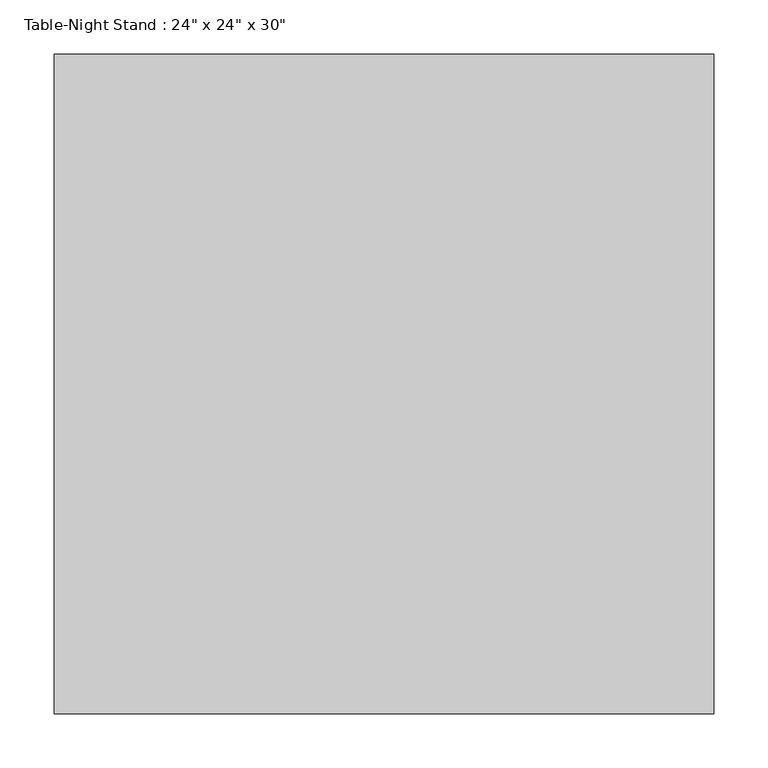
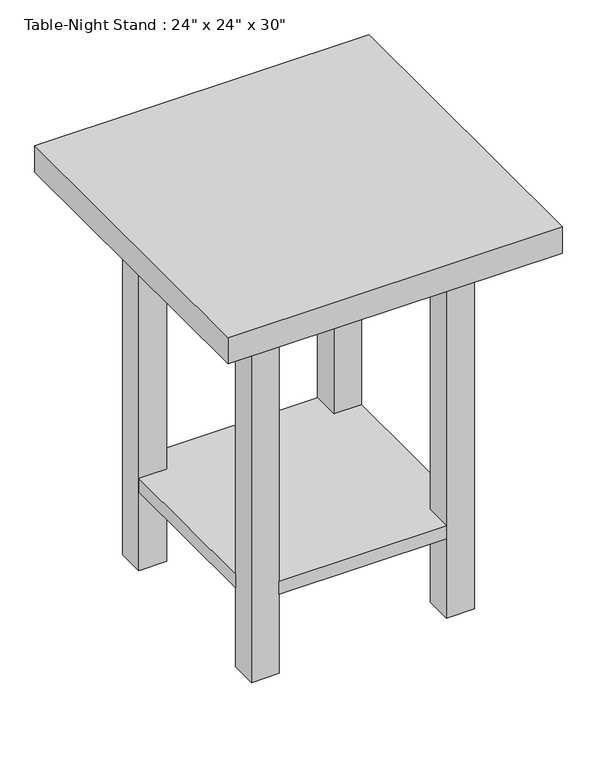
"""IFC4 building model written with IfcOpenShell, lengths in millimetres: furniture geometry."""

from ifc_helpers import new_model, si_unit, frame, origin, origin_with_axes, place, context, project, spatial, polyline, outline, extrude, source, transform, mapped, element, save


def furniture_5bc9ed15(model_context):
    return source(origin(), model_context, "Body", "SweptSolid", [
        extrude(outline(polyline([(156.1336303, 508.0), (460.9336303, 508.0), (460.9336303, 457.2), (511.7336303, 457.2), (511.7336303, 152.4), (460.9336303, 152.4), (460.9336303, 101.6), (156.1336303, 101.6), (156.1336303, 152.4), (105.3336303, 152.4), (105.3336303, 457.2), (156.1336303, 457.2), (156.1336303, 508.0)])), frame((0.0, 0.0, 152.4), z_axis=(0.0, 0.0, 1.0), x_axis=(1.0, 0.0, 0.0)), (0.0, 0.0, 1.0), 25.4),
        extrude(outline(polyline([(156.1336303, 508.0), (156.1336303, 457.2), (105.3336303, 457.2), (105.3336303, 508.0), (156.1336303, 508.0)])), origin_with_axes(), (0.0, 0.0, 1.0), 711.2),
        extrude(outline(polyline([(156.1336303, 152.4), (156.1336303, 101.6), (105.3336303, 101.6), (105.3336303, 152.4), (156.1336303, 152.4)])), origin_with_axes(), (0.0, 0.0, 1.0), 711.2),
        extrude(outline(polyline([(511.7336303, 508.0), (511.7336303, 457.2), (460.9336303, 457.2), (460.9336303, 508.0), (511.7336303, 508.0)])), origin_with_axes(), (0.0, 0.0, 1.0), 711.2),
        extrude(outline(polyline([(511.7336303, 152.4), (511.7336303, 101.6), (460.9336303, 101.6), (460.9336303, 152.4), (511.7336303, 152.4)])), origin_with_axes(), (0.0, 0.0, 1.0), 711.2),
        extrude(outline(polyline([(613.3336303, 0.0), (3.7336303, 0.0), (3.7336303, 609.6), (613.3336303, 609.6), (613.3336303, 0.0)])), frame((0.0, 0.0, 711.2), z_axis=(0.0, 0.0, 1.0), x_axis=(1.0, 0.0, 0.0)), (0.0, 0.0, 1.0), 50.8),
    ])


if __name__ == "__main__":
    model = new_model("IFC4")
    model_context = context("Model", 3, world=origin())
    ifc_project = project(units=[si_unit("LENGTHUNIT", "METRE", prefix="MILLI")], contexts=[model_context])
    site = spatial("IfcSite", under=ifc_project)
    building = spatial("IfcBuilding", under=site)
    placement = place(None, origin())
    furniture_shape = furniture_5bc9ed15(model_context)
    element("IfcFurniture", 1, ObjectType="Table-Night Stand : 24\" x 24\" x 30\"", at=placement, inside=building, context=model_context, shape_type="MappedRepresentation", body=[
        mapped(furniture_shape, transform((0.0, 0.0, 0.0), x_axis=(1.0, 0.0, 0.0), y_axis=(0.0, 1.0, 0.0), z_axis=(0.0, 0.0, 1.0))),
    ])
    save(model, "model.ifc")

# Revit data of these elements
# Type "Table-Night Stand : 24\" x 24\" x 30\""
#   Model = "Night Stand"
#   Manufacturer = "Acme Funriture"
#   Assembly Code = "E2020200"
#   Depth = 2' - 0"
#   Height = 2' - 6"
#   Width = 2' - 0"
#   Base Material = Birch
#   Top Material = Laminate, Blue, Matte
#   Default Elevation = 0
# Element 1 (IfcFurniture, "Table-Night Stand : 24\" x 24\" x 30\"")
#   Materials on its faces: "Birch", "Laminate, Blue, Matte"
# Materials
#   "Birch": class "Wood", colour RGB 172 132 95, transparency 0, Description = "Betula Alleghaniensis", Cost = 0
#   "Laminate, Blue, Matte": class "Plastic", colour RGB 85 101 155, transparency 0, Description = "Plastic Laminate - Blue, Matte", Cost = 0
